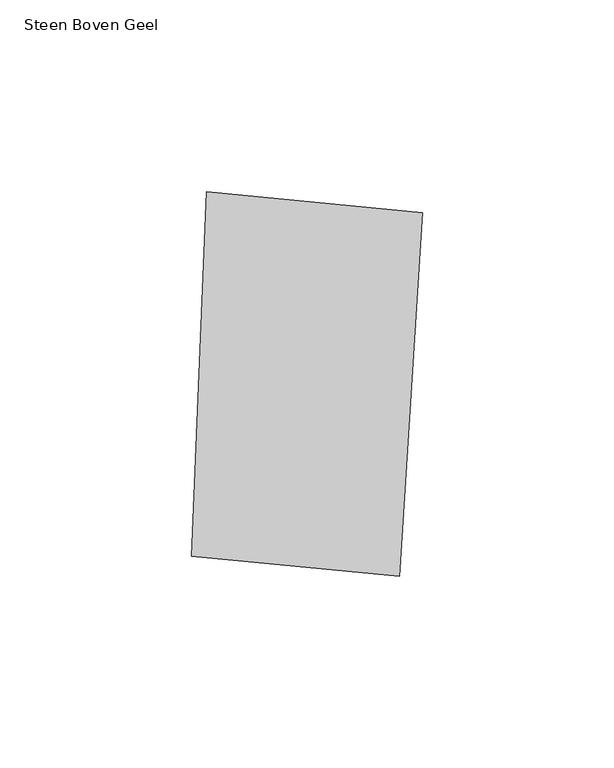
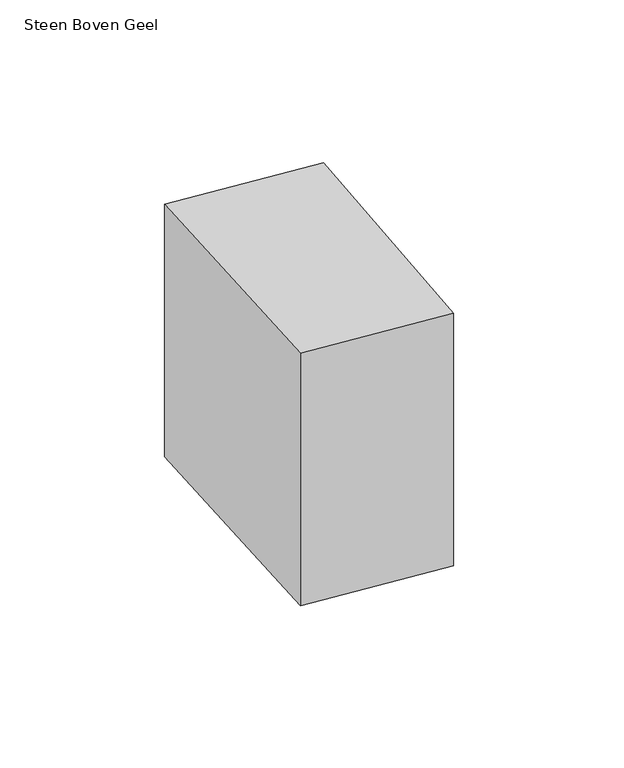
"""IFC4 building model written with IfcOpenShell, lengths in millimetres: proxy geometry, 00_GMA_steen_versie_4 : Steen Boven Geel."""

from ifc_helpers import new_model, si_unit, origin, origin_with_axes, place, context, project, spatial, polyline, outline, extrude, source, transform, mapped, element, save


def steen_boven_geel_6e8d8ada(model_context):
    return source(origin(), model_context, "Body", "SweptSolid", [
        extrude(outline(polyline([(103.7244962, 119.0056283), (97.7426982, 24.1381088), (43.439803, 29.3790697), (47.3203359, 124.4537309), (103.7244962, 119.0056283)])), origin_with_axes(), (0.0, 0.0, 1.0), 100.0),
    ])


if __name__ == "__main__":
    model = new_model("IFC4")
    model_context = context("Model", 3, world=origin())
    ifc_project = project(units=[si_unit("LENGTHUNIT", "METRE", prefix="MILLI")], contexts=[model_context])
    site = spatial("IfcSite", under=ifc_project)
    building = spatial("IfcBuilding", under=site)
    placement = place(None, origin())
    steen_boven_geel_shape = steen_boven_geel_6e8d8ada(model_context)
    element("IfcBuildingElementProxy", 1, Name="00_GMA_steen_versie_4 : Steen Boven Geel", ObjectType="00_GMA_steen_versie_4 : Steen Boven Geel", at=placement, inside=building, context=model_context, shape_type="MappedRepresentation", body=[
        mapped(steen_boven_geel_shape, transform((0.0, 0.0, 0.0), x_axis=(1.0, 0.0, 0.0), y_axis=(0.0, 1.0, 0.0), z_axis=(0.0, 0.0, 1.0))),
    ])
    save(model, "model.ifc")

# Revit data of these elements
# Type "00_GMA_steen_versie_4 : Steen Boven Geel"
#   StootVoegHalfBoven [instance default] = 5 mm
#   StootVoegHalf [instance default] = 5 mm
#   StootVoegBreedteOnder = 10 mm
#   StootVoegBreedteBoven = 10 mm
#   Steendikte = 100 mm
#   LintVoegOnderHalf = 5 mm
#   LintVoegOnder = 10 mm
#   LintVoegBovenHalf = 0 mm
#   LintVoegBoven = 0 mm
#   materiaal = 21_steen_geel
#   MateriaalVoeg = none
#   Default Elevation = 0
# Element 1 (IfcBuildingElementProxy, "00_GMA_steen_versie_4 : Steen Boven Geel")
#   Materials on its faces: "21_steen_geel"
# Materials
#   "21_steen_geel": class "Unassigned", colour RGB 202 202 0, transparency 0, Cost = 0
